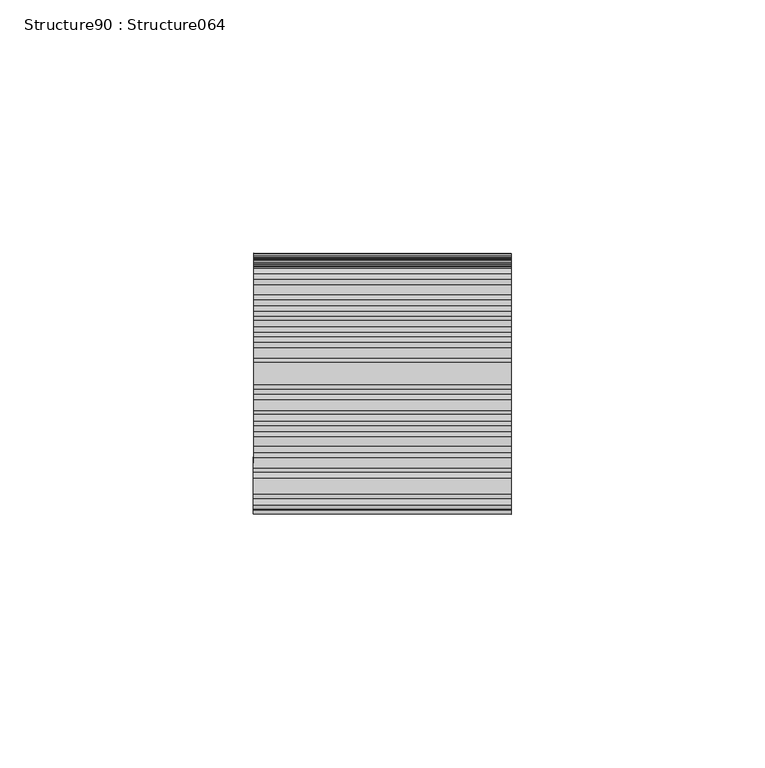
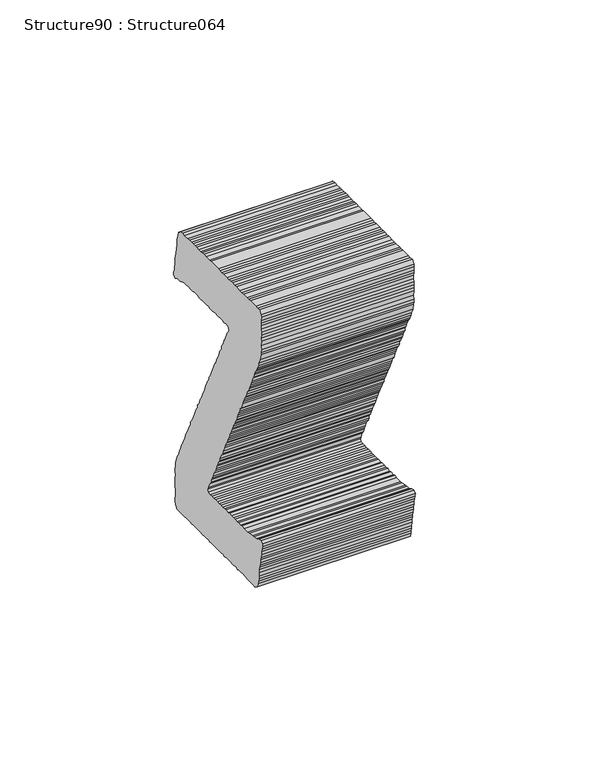
"""IFC4 building model written with IfcOpenShell, lengths in millimetres: proxy geometry, Structure90 : Structure064."""

import ifcopenshell
import ifcopenshell.guid

model = None  # the IFC model being written
_history = None  # IfcOwnerHistory: only IFC2X3 demands one
_inside = {}  # id of a spatial element -> (the spatial element, [elements in it])
_under = {}  # id of a project, library or spatial element -> (it, [spatial elements below it])
_declared = {}  # id of a project -> (the project, [libraries it declares])
_typed = {}  # id of a type object -> (the type object, [elements of that type])
_made_of = {}  # id of a material, layer set ... -> (it, [elements and type objects made of it])


def new_model(schema):
    """Start an empty IFC model of exactly this schema.

    Asked for "IFC4X3", IfcOpenShell would pick the latest addendum, in which some entities
    have other attributes; the version numbers below select the first issue.
    IFC2X3 requires an IfcOwnerHistory on every rooted entity: one is made here for all.
    """
    global model, _history
    if schema == "IFC4X3":
        model = ifcopenshell.file(schema_version=(4, 3, 0, 0))
    else:
        model = ifcopenshell.file(schema=schema)
    _inside.clear()
    _under.clear()
    _declared.clear()
    _typed.clear()
    _made_of.clear()
    _history = None
    if model.schema == "IFC2X3":
        org = make("IfcOrganization", Name="unknown")
        user = make(
            "IfcPersonAndOrganization",
            ThePerson=make("IfcPerson", FamilyName="unknown"),
            TheOrganization=org,
        )
        app = make(
            "IfcApplication",
            ApplicationDeveloper=org,
            Version="unknown",
            ApplicationFullName="unknown",
            ApplicationIdentifier="unknown",
        )
        _history = make(
            "IfcOwnerHistory",
            OwningUser=user,
            OwningApplication=app,
            ChangeAction="ADDED",
            CreationDate=0,
        )
    return model


def make(cls, **values):
    """One entity of the class cls with the attributes given. An attribute that is None is left unset."""
    return model.create_entity(
        cls, **{name: value for name, value in values.items() if value is not None}
    )


def rooted(cls, **values):
    """An entity with a GlobalId (a new one), such as an element, a storey or a relation."""
    return make(cls, GlobalId=ifcopenshell.guid.new(), OwnerHistory=_history, **values)


def si_unit(unit_type, name, prefix=None):
    """IfcSIUnit, for example si_unit("LENGTHUNIT", "METRE", prefix="MILLI")."""
    return make("IfcSIUnit", UnitType=unit_type, Prefix=prefix, Name=name)


def assignment(units):
    """IfcUnitAssignment: the units of a project."""
    return None if units is None else make("IfcUnitAssignment", Units=units)


def point(xyz):
    """IfcCartesianPoint."""
    return None if xyz is None else make("IfcCartesianPoint", Coordinates=xyz)


def direction(xyz):
    """IfcDirection."""
    return None if xyz is None else make("IfcDirection", DirectionRatios=xyz)


def frame(location, z_axis=None, x_axis=None):
    """IfcAxis2Placement3D, a coordinate frame: its origin and axes. An axis left out is left unset."""
    return make(
        "IfcAxis2Placement3D",
        Location=point(location),
        Axis=direction(z_axis),
        RefDirection=direction(x_axis),
    )


def origin():
    """The frame at (0, 0, 0) with its axes left unset."""
    return frame((0.0, 0.0, 0.0))


def place(relative_to, where):
    """IfcLocalPlacement: puts the frame where relative to a parent placement (None: the world)."""
    return make(
        "IfcLocalPlacement", PlacementRelTo=relative_to, RelativePlacement=where
    )


def context(
    kind, dimensions, precision=None, world=None, true_north=None, identifier=None
):
    """IfcGeometricRepresentationContext, for example the 3D "Model" context."""
    return make(
        "IfcGeometricRepresentationContext",
        ContextIdentifier=identifier,
        ContextType=kind,
        CoordinateSpaceDimension=dimensions,
        Precision=precision,
        WorldCoordinateSystem=world,
        TrueNorth=true_north,
    )


def project(units=None, contexts=None):
    """IfcProject with its units and contexts."""
    return rooted(
        "IfcProject",
        Name="project",
        RepresentationContexts=contexts,
        UnitsInContext=assignment(units),
    )


def spatial(cls, under=None, at=None, **own):
    """A site, building, storey or space (cls), placed at a placement, below another one or the project."""
    s = rooted(cls, ObjectPlacement=at, **own)
    if under is not None:
        _under.setdefault(under.id(), (under, []))[1].append(s)
    return s


def polyline(points):
    """IfcPolyline through the points."""
    return make("IfcPolyline", Points=[point(p) for p in points])


def outline(outer, holes=None, kind="AREA"):
    """IfcArbitraryClosedProfileDef: a profile drawn as a closed curve; with holes, ...WithVoids."""
    if holes is None:
        return make("IfcArbitraryClosedProfileDef", ProfileType=kind, OuterCurve=outer)
    return make(
        "IfcArbitraryProfileDefWithVoids",
        ProfileType=kind,
        OuterCurve=outer,
        InnerCurves=holes,
    )


def extrude(swept, where, along, depth):
    """IfcExtrudedAreaSolid: the profile swept, set in the frame where, extruded along a direction by depth."""
    return make(
        "IfcExtrudedAreaSolid",
        SweptArea=swept,
        Position=where,
        ExtrudedDirection=direction(along),
        Depth=depth,
    )


def shape(context_of_items, identifier, shape_type, items):
    """IfcShapeRepresentation: the items that make up one representation, for example the "Body"."""
    return make(
        "IfcShapeRepresentation",
        ContextOfItems=context_of_items,
        RepresentationIdentifier=identifier,
        RepresentationType=shape_type,
        Items=items,
    )


def source(mapping_origin, context_of_items, identifier, shape_type, items):
    """IfcRepresentationMap: a shape defined once, which mapped items show again and again."""
    return make(
        "IfcRepresentationMap",
        MappingOrigin=mapping_origin,
        MappedRepresentation=shape(context_of_items, identifier, shape_type, items),
    )


def transform(
    local_origin,
    x_axis=None,
    y_axis=None,
    z_axis=None,
    scale=None,
    scale2=None,
    scale3=None,
    uniform=True,
):
    """IfcCartesianTransformationOperator3D, or its non-uniform kind. x_axis, y_axis, z_axis: its Axis1, 2, 3."""
    if uniform:
        return make(
            "IfcCartesianTransformationOperator3D",
            Axis1=direction(x_axis),
            Axis2=direction(y_axis),
            LocalOrigin=point(local_origin),
            Scale=scale,
            Axis3=direction(z_axis),
        )
    return make(
        "IfcCartesianTransformationOperator3DnonUniform",
        Axis1=direction(x_axis),
        Axis2=direction(y_axis),
        LocalOrigin=point(local_origin),
        Scale=scale,
        Axis3=direction(z_axis),
        Scale2=scale2,
        Scale3=scale3,
    )


def mapped(mapping_source, mapping_target):
    """IfcMappedItem: shows the shape of a source again, moved by a transform."""
    return make(
        "IfcMappedItem", MappingSource=mapping_source, MappingTarget=mapping_target
    )


def made_of(thing, what):
    """Note that an element or type object is made of a material, layer set ...; save() writes the relation."""
    if what is not None:
        _made_of.setdefault(what.id(), (what, []))[1].append(thing)
    return thing


def element(
    cls,
    number,
    at=None,
    inside=None,
    cuts=None,
    type_object=None,
    material=None,
    context=None,
    identifier="Body",
    shape_type=None,
    held_by="IfcProductDefinitionShape",
    body=None,
    shapes=None,
    **own,
):
    """One element of the class cls, such as IfcWall. Its Tag is "e" and its number.

    at: its placement. inside: the storey or other place that contains it. cuts: it is an
    opening in that element (IfcRelVoidsElement). A single representation is given by context,
    identifier, shape_type and body (its items); several are given by shapes. held_by: the class
    of the entity that holds the representations. save() writes the other relations.
    """
    e = rooted(cls, Tag="e%d" % number, ObjectPlacement=at, **own)
    if body is not None:
        shapes = [shape(context, identifier, shape_type, body)]
    if shapes is not None:
        e.Representation = make(held_by, Representations=shapes)
    if inside is not None:
        _inside.setdefault(inside.id(), (inside, []))[1].append(e)
    if cuts is not None:
        rooted(
            "IfcRelVoidsElement", RelatingBuildingElement=cuts, RelatedOpeningElement=e
        )
    if type_object is not None:
        _typed.setdefault(type_object.id(), (type_object, []))[1].append(e)
    return made_of(e, material)


def aggregate(whole, parts):
    """IfcRelAggregates: a whole, such as a stair, and the parts it consists of."""
    return rooted("IfcRelAggregates", RelatingObject=whole, RelatedObjects=parts)


def save(model, path):
    """Write the relations noted so far, then the file.

    IfcRelAggregates (storeys below a building ...), IfcRelContainedInSpatialStructure (elements
    in a storey), IfcRelDefinesByType, IfcRelAssociatesMaterial and IfcRelDeclares: one each for
    every whole, place, type object, material and project.
    """
    for whole, parts in _under.values():
        aggregate(whole, parts)
    for where, things in _inside.values():
        rooted(
            "IfcRelContainedInSpatialStructure",
            RelatedElements=things,
            RelatingStructure=where,
        )
    for kind, things in _typed.values():
        rooted("IfcRelDefinesByType", RelatedObjects=things, RelatingType=kind)
    for what, things in _made_of.values():
        rooted("IfcRelAssociatesMaterial", RelatedObjects=things, RelatingMaterial=what)
    for by, libraries in _declared.values():
        rooted("IfcRelDeclares", RelatingContext=by, RelatedDefinitions=libraries)
    model.write(path)


def structure90_structure064_e0061a47(model_context):
    return source(origin(), model_context, "Body", "SweptSolid", [
        extrude(outline(polyline([(1.0468911, 0.0), (1.5156229, -1.0820274), (1.804305, -2.1128067), (2.0901184, -3.1435852), (2.6051551, -4.0455173), (2.8493861, -5.2553333), (3.1877266, -6.1090195), (3.6541637, -7.1898987), (3.9427132, -8.2211635), (4.2191678, -8.9614524), (4.5077173, -9.9927171), (4.9123564, -10.9617879), (5.4407689, -12.1519159), (5.8915804, -12.9413769), (6.1839247, -13.9749819), (6.5222652, -14.828668), (6.9380301, -16.0827122), (6.1506864, -17.5841228), (5.2932054, -17.920123), (4.5699105, -18.4868046), (2.5398679, -19.6460344), (0.6051261, -20.450503), (-0.1861888, -20.9023732), (-1.1371166, -21.592076), (-2.1040692, -21.9975542), (-2.6501814, -22.6097455), (-3.6829911, -22.8991774), (-4.680224, -23.7689753), (-6.7289819, -24.6385514), (-8.420375, -25.6043997), (-9.1948285, -26.3469823), (-10.1136221, -26.5713067), (-10.9983838, -27.3768795), (-12.014332, -27.9570237), (-12.9842842, -28.3572492), (-14.6772222, -29.3239797), (-15.754483, -29.7924481), (-16.4146114, -30.4697468), (-17.3352589, -30.6951299), (-18.3324918, -31.5649279), (-19.3021349, -31.9649769), (-20.2522261, -32.6611675), (-21.2200153, -33.0601579), (-24.6065095, -34.9939719), (-25.6665998, -35.7529762), (-26.4100647, -36.023869), (-28.329799, -37.1201087), (-29.1634022, -37.7497804), (-31.7601263, -39.2326064), (-32.9547118, -39.7611059), (-34.3223761, -39.1993681), (-35.0653556, -38.4235023), (-35.5144027, -37.6371312), (-35.8683687, -36.4920267), (-36.4973321, -35.6510535), (-37.0123689, -34.7491213), (-37.5131478, -34.13693), (-39.0600225, -31.4280437), (-39.3479989, -30.3985003), (-40.2164292, -29.4029449), (-40.6060152, -28.7207023), (-41.0222655, -27.4665256), (-41.5390667, -26.5615036), (-41.9878048, -24.7280648), (-42.0390503, -23.8526173), (-42.0359182, -22.8104935), (-42.2127016, -21.7108988), (-42.4538004, -20.5058502), (-42.3247311, -19.6806798), (-42.5689621, -18.470864), (-42.7916546, -17.5556456), (-42.5507769, -16.6686772), (-42.8556577, -15.3447582), (-42.7933303, -13.3637113), (-43.1941746, -12.3969807), (-43.3090273, -10.3618179), (-43.1942185, -9.2555128), (-43.3048358, -8.2717882), (-43.3060717, -7.2256028), (-43.3026728, -6.1767707), (-43.7729495, -5.0956256), (-43.6411896, -4.2758844), (-43.7089007, -3.1140055), (-43.7694181, -1.9525258), (-43.9492913, 0.1921955), (-44.0598215, 1.1714626), (-44.1720706, 2.1587625), (-44.0444594, 2.9785932), (-44.3984253, 4.1236976), (-44.2202735, 5.1190766), (-44.2861307, 6.2820142), (-44.510455, 7.2008078), (-44.5086906, 8.244609), (-44.5569365, 9.1148039), (-44.7333238, 10.2101174), (-44.6853413, 11.4384715), (-44.8615523, 12.533476), (-44.9124887, 13.4091), (-45.202319, 14.4375847), (-45.1999796, 15.485402), (-45.2642048, 16.6447643), (-45.2012147, 18.6282384), (-45.4706529, 19.3655683), (-45.4880876, 20.7048933), (-45.4254066, 21.6412998), (-45.6497308, 22.5600935), (-45.7639234, 23.5421861), (-45.7771226, 24.8769642), (-45.8922843, 25.8650592), (-46.0677895, 26.9588279), (-45.8232495, 27.8429708), (-46.1799516, 28.9885614), (-46.1609712, 30.7936608), (-46.2269608, 31.956113), (-46.5805308, 33.0969364), (-46.5805308, 34.1438276), (-46.4040109, 35.1427817), (-46.8050315, 36.1098213), (-46.8077222, 37.1621417), (-46.690883, 38.2691965), (-47.0972434, 39.237694), (-46.9643793, 40.0605242), (-47.1443851, 41.157869), (-47.093712, 42.3807938), (-47.2075516, 43.3622686), (-47.1442526, 44.2990279), (-47.1397519, 45.3423429), (-48.2212035, 45.927387), (-49.2535278, 45.6378228), (-50.1403199, 44.8315002), (-51.1714082, 44.5426417), (-51.9611782, 44.0916537), (-52.7336451, 43.3506151), (-53.52496, 42.8987449), (-54.6697555, 42.5449553), (-55.2837113, 42.0472663), (-56.1182853, 41.4178597), (-57.1339245, 40.8378919), (-58.0543956, 40.6122), (-58.7808227, 40.0502857), (-59.908933, 39.4060927), (-60.5188737, 38.9049601), (-62.438299, 37.8088969), (-63.5815495, 37.4559896), (-65.1620164, 36.5534843), (-65.9366463, 35.8112105), (-66.7264163, 35.3602225), (-67.982138, 34.94309), (-68.6436787, 34.2653944), (-70.2229097, 33.3635947), (-71.0918685, 32.2691635), (-71.7529686, 31.5892611), (-72.5914252, 30.9637834), (-73.3161772, 30.3946308), (-73.9653562, 29.4326676), (-75.1394627, 29.655447), (-75.5424242, 30.6258854), (-75.6545864, 31.6087278), (-75.9436214, 32.6401252), (-76.4771971, 33.831402), (-76.7505171, 34.5755297), (-77.391887, 35.6986963), (-77.7957308, 36.6706796), (-77.9533158, 37.4718819), (-78.7142154, 39.5872052), (-78.9373933, 40.5025561), (-79.5203606, 41.5234481), (-79.9227498, 42.4892965), (-80.2107261, 43.5188399), (-80.3734288, 44.3261341), (-80.7886205, 45.5784569), (-80.2754789, 46.7786489), (-79.3887764, 47.5808228), (-78.3594524, 47.8727712), (-76.6646605, 48.8405604), (-75.891974, 49.577627), (-74.8114916, 50.0454765), (-73.9725487, 50.6736902), (-73.0703076, 51.1889034), (-72.3272387, 51.4640773), (-71.1375066, 51.9967708), (-70.2343385, 52.5125134), (-69.5077351, 53.0741187), (-68.6700282, 53.7016266), (-67.5898547, 54.1692997), (-65.7862995, 55.1991968), (-65.1716809, 55.6993129), (-61.3380831, 57.8884398), (-60.482234, 58.2280154), (-59.6296064, 58.5682097), (-58.74105, 59.3714423), (-56.9374946, 60.4013395), (-56.1324951, 60.5651903), (-55.1302315, 61.4333539), (-54.3407705, 61.8841655), (-53.2624511, 62.3507799), (-52.4228901, 62.9793465), (-50.7144135, 63.6591163), (-49.587848, 64.3024271), (-48.7478465, 64.928787), (-46.9439823, 65.9588605), (-46.2038259, 66.2348296), (-45.3152694, 67.0380622), (-42.607928, 68.5840548), (-41.6907663, 68.8119544), (-40.6881938, 69.6802944), (-39.4295156, 69.0489461), (-38.8664093, 68.3240193), (-38.3978541, 67.242301), (-37.9496891, 66.4574748), (-37.5491538, 65.4905678), (-36.9661865, 64.4696758), (-36.2903432, 63.8128137), (-35.7761886, 62.9124265), (-35.3048103, 61.8257644), (-34.6803019, 60.9933102), (-34.0695237, 59.3970413), (-33.261701, 58.5090571), (-32.7927929, 57.4267209), (-32.5233546, 56.689391), (-31.8933327, 54.7996726), (-31.7828479, 52.7685714), (-31.3793545, 51.8058121), (-31.3631118, 50.4649869), (-31.3171157, 49.5980145), (-31.4264548, 48.4821308), (-31.3141161, 47.4989794), (-31.3141162, 46.4520882), (-31.0267578, 45.422192), (-31.2049097, 44.4268131), (-30.8021245, 43.4566837), (-30.7842044, 42.1172261), (-30.6228701, 41.3087407), (-30.5595711, 40.1517178), (-30.5105754, 39.2794926), (-30.3833162, 38.0090276), (-30.6263112, 37.1257669), (-30.2862072, 36.2661223), (-30.1608458, 34.9953931), (-30.3373657, 33.9964388), (-30.2234822, 33.0141697), (-30.0459931, 31.9133391), (-29.9811051, 30.7564039), (-29.5819384, 28.7414145), (-29.9381551, 27.7930903), (-29.6441332, 26.760853), (-29.5336485, 25.776643), (-29.5176692, 24.4405844), (-29.3570847, 23.6341293), (-29.1790199, 22.5401834), (-29.291713, 21.4244331), (-29.1327604, 20.6215534), (-29.1349233, 19.5734271), (-29.1347468, 18.526227), (-28.9548737, 17.4283968), (-29.0688898, 16.3163981), (-28.7320943, 15.4618297), (-28.8282772, 14.0617224), (-28.6024078, 13.1438109), (-28.602012, 12.0926387), (-28.5377867, 10.9332764), (-28.4256246, 9.950434), (-28.4919232, 9.0189274), (-28.2493697, 7.8077438), (-28.2512236, 6.759794), (-28.0397895, 5.0821725), (-27.8495403, 3.7013993), (-27.9605568, 2.5841479), (-27.8483947, 0.5544144), (-27.5760439, -0.1837108), (-27.7373342, -1.4698022), (-27.5098777, -2.3933631), (-27.6243354, -3.5060236), (-27.2216372, -4.4716955), (-27.1105345, -5.4555526), (-27.2876724, -7.5017509), (-27.0481185, -8.7076817), (-26.9810702, -9.8719878), (-26.9826152, -10.9197612), (-26.6425533, -11.7728741), (-26.807419, -13.0605974), (-26.5826092, -15.0264147), (-26.4179656, -15.8371077), (-25.8082014, -16.3825572), (-24.7266594, -15.913693), (-23.775069, -15.221563), (-22.9231041, -14.8837959), (-22.020863, -14.3685826), (-21.0674186, -13.675394), (-20.1480517, -13.4527911), (-19.3104318, -12.8208257), (-18.5688208, -12.5509915), (-17.6208925, -11.8560359), (-16.8936264, -11.2920035), (-15.6368461, -10.876725), (-15.0882172, -10.2610477), (-14.0100742, -9.7941244), (-13.106288, -9.2780289), (-12.2668598, -8.6499477), (-11.2365667, -8.3640018), (-10.625434, -7.861369), (-9.4293035, -7.3319873), (-8.7697485, -6.6529671), (-7.7363655, -6.3652567), (-5.9325012, -5.3351832), (-5.15893, -4.5910555), (-3.5987235, -3.3997786), (-2.9839284, -2.8999714), (-1.9218076, -2.1402174), (-1.3699598, -1.533765), (-0.8395608, -0.6285666), (0.0, 0.0), (1.0468911, 0.0)])), frame((-56111.1833189, 291992.6126506, -357.1515075), z_axis=(-0.9999998917542983, 0.0004652863545059615, 0.0), x_axis=(-0.000404049791022153, -0.8683894194936091, -0.4958827007018082)), (0.0, 0.0, 1.0), 50.8),
    ])


if __name__ == "__main__":
    model = new_model("IFC4")
    model_context = context("Model", 3, world=origin())
    ifc_project = project(units=[si_unit("LENGTHUNIT", "METRE", prefix="MILLI")], contexts=[model_context])
    site = spatial("IfcSite", under=ifc_project)
    building = spatial("IfcBuilding", under=site)
    placement = place(None, origin())
    structure90_structure064_shape = structure90_structure064_e0061a47(model_context)
    element("IfcBuildingElementProxy", 1, Name="Structure90 : Structure064", ObjectType="Structure90 : Structure064", at=placement, inside=building, context=model_context, shape_type="MappedRepresentation", body=[
        mapped(structure90_structure064_shape, transform((0.0, 0.0, 0.0), x_axis=(1.0, 0.0, 0.0), y_axis=(0.0, 1.0, 0.0), z_axis=(0.0, 0.0, 1.0))),
    ])
    save(model, "model.ifc")

# Revit data of these elements
# Type "Structure90 : Structure064"
#   NameOverride = "Structure064"
# Element 1 (IfcBuildingElementProxy, "Structure90 : Structure064")
#   Materials on its faces: "BRUSHED ALUMINUM LETTERING"
# Materials
#   "BRUSHED ALUMINUM LETTERING": class "Unassigned", colour RGB 169 181 186, transparency 0, Cost = 0
